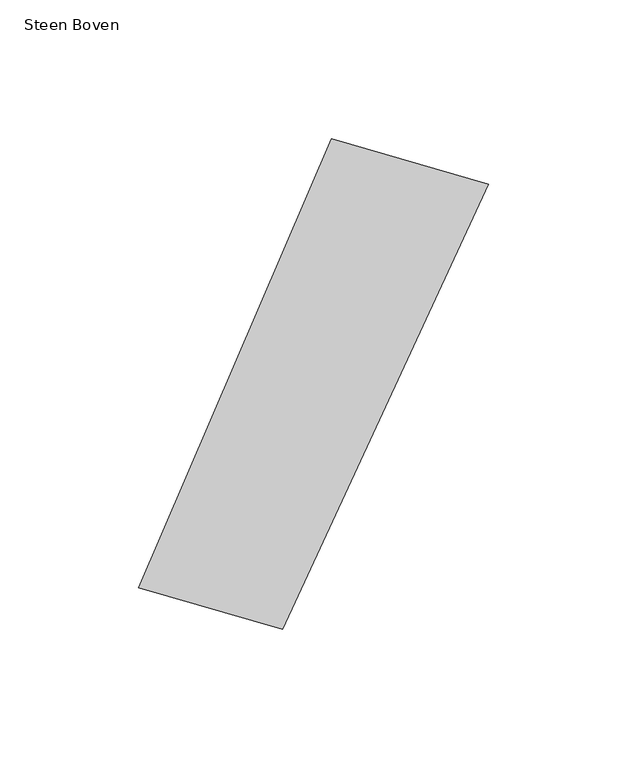
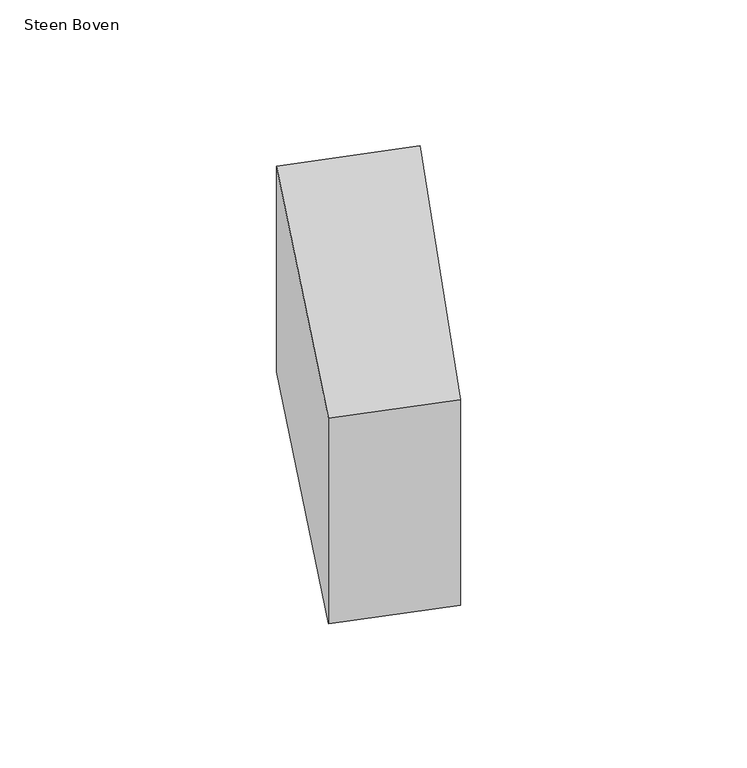
"""IFC4 building model written with IfcOpenShell, lengths in millimetres: proxy geometry, 00_GMA_steen_versie_4 : Steen Boven."""

import ifcopenshell
import ifcopenshell.guid

model = None  # the IFC model being written
_history = None  # IfcOwnerHistory: only IFC2X3 demands one
_inside = {}  # id of a spatial element -> (the spatial element, [elements in it])
_under = {}  # id of a project, library or spatial element -> (it, [spatial elements below it])
_declared = {}  # id of a project -> (the project, [libraries it declares])
_typed = {}  # id of a type object -> (the type object, [elements of that type])
_made_of = {}  # id of a material, layer set ... -> (it, [elements and type objects made of it])


def new_model(schema):
    """Start an empty IFC model of exactly this schema.

    Asked for "IFC4X3", IfcOpenShell would pick the latest addendum, in which some entities
    have other attributes; the version numbers below select the first issue.
    IFC2X3 requires an IfcOwnerHistory on every rooted entity: one is made here for all.
    """
    global model, _history
    if schema == "IFC4X3":
        model = ifcopenshell.file(schema_version=(4, 3, 0, 0))
    else:
        model = ifcopenshell.file(schema=schema)
    _inside.clear()
    _under.clear()
    _declared.clear()
    _typed.clear()
    _made_of.clear()
    _history = None
    if model.schema == "IFC2X3":
        org = make("IfcOrganization", Name="unknown")
        user = make(
            "IfcPersonAndOrganization",
            ThePerson=make("IfcPerson", FamilyName="unknown"),
            TheOrganization=org,
        )
        app = make(
            "IfcApplication",
            ApplicationDeveloper=org,
            Version="unknown",
            ApplicationFullName="unknown",
            ApplicationIdentifier="unknown",
        )
        _history = make(
            "IfcOwnerHistory",
            OwningUser=user,
            OwningApplication=app,
            ChangeAction="ADDED",
            CreationDate=0,
        )
    return model


def make(cls, **values):
    """One entity of the class cls with the attributes given. An attribute that is None is left unset."""
    return model.create_entity(
        cls, **{name: value for name, value in values.items() if value is not None}
    )


def rooted(cls, **values):
    """An entity with a GlobalId (a new one), such as an element, a storey or a relation."""
    return make(cls, GlobalId=ifcopenshell.guid.new(), OwnerHistory=_history, **values)


def si_unit(unit_type, name, prefix=None):
    """IfcSIUnit, for example si_unit("LENGTHUNIT", "METRE", prefix="MILLI")."""
    return make("IfcSIUnit", UnitType=unit_type, Prefix=prefix, Name=name)


def assignment(units):
    """IfcUnitAssignment: the units of a project."""
    return None if units is None else make("IfcUnitAssignment", Units=units)


def point(xyz):
    """IfcCartesianPoint."""
    return None if xyz is None else make("IfcCartesianPoint", Coordinates=xyz)


def direction(xyz):
    """IfcDirection."""
    return None if xyz is None else make("IfcDirection", DirectionRatios=xyz)


def frame(location, z_axis=None, x_axis=None):
    """IfcAxis2Placement3D, a coordinate frame: its origin and axes. An axis left out is left unset."""
    return make(
        "IfcAxis2Placement3D",
        Location=point(location),
        Axis=direction(z_axis),
        RefDirection=direction(x_axis),
    )


def origin():
    """The frame at (0, 0, 0) with its axes left unset."""
    return frame((0.0, 0.0, 0.0))


def origin_with_axes():
    """The frame at (0, 0, 0) with the z axis (0, 0, 1) and the x axis (1, 0, 0) written out."""
    return frame((0.0, 0.0, 0.0), z_axis=(0.0, 0.0, 1.0), x_axis=(1.0, 0.0, 0.0))


def place(relative_to, where):
    """IfcLocalPlacement: puts the frame where relative to a parent placement (None: the world)."""
    return make(
        "IfcLocalPlacement", PlacementRelTo=relative_to, RelativePlacement=where
    )


def context(
    kind, dimensions, precision=None, world=None, true_north=None, identifier=None
):
    """IfcGeometricRepresentationContext, for example the 3D "Model" context."""
    return make(
        "IfcGeometricRepresentationContext",
        ContextIdentifier=identifier,
        ContextType=kind,
        CoordinateSpaceDimension=dimensions,
        Precision=precision,
        WorldCoordinateSystem=world,
        TrueNorth=true_north,
    )


def project(units=None, contexts=None):
    """IfcProject with its units and contexts."""
    return rooted(
        "IfcProject",
        Name="project",
        RepresentationContexts=contexts,
        UnitsInContext=assignment(units),
    )


def spatial(cls, under=None, at=None, **own):
    """A site, building, storey or space (cls), placed at a placement, below another one or the project."""
    s = rooted(cls, ObjectPlacement=at, **own)
    if under is not None:
        _under.setdefault(under.id(), (under, []))[1].append(s)
    return s


def polyline(points):
    """IfcPolyline through the points."""
    return make("IfcPolyline", Points=[point(p) for p in points])


def outline(outer, holes=None, kind="AREA"):
    """IfcArbitraryClosedProfileDef: a profile drawn as a closed curve; with holes, ...WithVoids."""
    if holes is None:
        return make("IfcArbitraryClosedProfileDef", ProfileType=kind, OuterCurve=outer)
    return make(
        "IfcArbitraryProfileDefWithVoids",
        ProfileType=kind,
        OuterCurve=outer,
        InnerCurves=holes,
    )


def extrude(swept, where, along, depth):
    """IfcExtrudedAreaSolid: the profile swept, set in the frame where, extruded along a direction by depth."""
    return make(
        "IfcExtrudedAreaSolid",
        SweptArea=swept,
        Position=where,
        ExtrudedDirection=direction(along),
        Depth=depth,
    )


def shape(context_of_items, identifier, shape_type, items):
    """IfcShapeRepresentation: the items that make up one representation, for example the "Body"."""
    return make(
        "IfcShapeRepresentation",
        ContextOfItems=context_of_items,
        RepresentationIdentifier=identifier,
        RepresentationType=shape_type,
        Items=items,
    )


def source(mapping_origin, context_of_items, identifier, shape_type, items):
    """IfcRepresentationMap: a shape defined once, which mapped items show again and again."""
    return make(
        "IfcRepresentationMap",
        MappingOrigin=mapping_origin,
        MappedRepresentation=shape(context_of_items, identifier, shape_type, items),
    )


def transform(
    local_origin,
    x_axis=None,
    y_axis=None,
    z_axis=None,
    scale=None,
    scale2=None,
    scale3=None,
    uniform=True,
):
    """IfcCartesianTransformationOperator3D, or its non-uniform kind. x_axis, y_axis, z_axis: its Axis1, 2, 3."""
    if uniform:
        return make(
            "IfcCartesianTransformationOperator3D",
            Axis1=direction(x_axis),
            Axis2=direction(y_axis),
            LocalOrigin=point(local_origin),
            Scale=scale,
            Axis3=direction(z_axis),
        )
    return make(
        "IfcCartesianTransformationOperator3DnonUniform",
        Axis1=direction(x_axis),
        Axis2=direction(y_axis),
        LocalOrigin=point(local_origin),
        Scale=scale,
        Axis3=direction(z_axis),
        Scale2=scale2,
        Scale3=scale3,
    )


def mapped(mapping_source, mapping_target):
    """IfcMappedItem: shows the shape of a source again, moved by a transform."""
    return make(
        "IfcMappedItem", MappingSource=mapping_source, MappingTarget=mapping_target
    )


def made_of(thing, what):
    """Note that an element or type object is made of a material, layer set ...; save() writes the relation."""
    if what is not None:
        _made_of.setdefault(what.id(), (what, []))[1].append(thing)
    return thing


def element(
    cls,
    number,
    at=None,
    inside=None,
    cuts=None,
    type_object=None,
    material=None,
    context=None,
    identifier="Body",
    shape_type=None,
    held_by="IfcProductDefinitionShape",
    body=None,
    shapes=None,
    **own,
):
    """One element of the class cls, such as IfcWall. Its Tag is "e" and its number.

    at: its placement. inside: the storey or other place that contains it. cuts: it is an
    opening in that element (IfcRelVoidsElement). A single representation is given by context,
    identifier, shape_type and body (its items); several are given by shapes. held_by: the class
    of the entity that holds the representations. save() writes the other relations.
    """
    e = rooted(cls, Tag="e%d" % number, ObjectPlacement=at, **own)
    if body is not None:
        shapes = [shape(context, identifier, shape_type, body)]
    if shapes is not None:
        e.Representation = make(held_by, Representations=shapes)
    if inside is not None:
        _inside.setdefault(inside.id(), (inside, []))[1].append(e)
    if cuts is not None:
        rooted(
            "IfcRelVoidsElement", RelatingBuildingElement=cuts, RelatedOpeningElement=e
        )
    if type_object is not None:
        _typed.setdefault(type_object.id(), (type_object, []))[1].append(e)
    return made_of(e, material)


def aggregate(whole, parts):
    """IfcRelAggregates: a whole, such as a stair, and the parts it consists of."""
    return rooted("IfcRelAggregates", RelatingObject=whole, RelatedObjects=parts)


def save(model, path):
    """Write the relations noted so far, then the file.

    IfcRelAggregates (storeys below a building ...), IfcRelContainedInSpatialStructure (elements
    in a storey), IfcRelDefinesByType, IfcRelAssociatesMaterial and IfcRelDeclares: one each for
    every whole, place, type object, material and project.
    """
    for whole, parts in _under.values():
        aggregate(whole, parts)
    for where, things in _inside.values():
        rooted(
            "IfcRelContainedInSpatialStructure",
            RelatedElements=things,
            RelatingStructure=where,
        )
    for kind, things in _typed.values():
        rooted("IfcRelDefinesByType", RelatedObjects=things, RelatingType=kind)
    for what, things in _made_of.values():
        rooted("IfcRelAssociatesMaterial", RelatedObjects=things, RelatingMaterial=what)
    for by, libraries in _declared.values():
        rooted("IfcRelDeclares", RelatingContext=by, RelatedDefinitions=libraries)
    model.write(path)


def steen_boven_c7bab40e(model_context):
    return source(origin(), model_context, "Body", "SweptSolid", [
        extrude(outline(polyline([(138.9626949, 152.6124457), (64.6394864, -8.0916632), (12.6572251, 7.0193553), (82.3362997, 169.0557906), (138.9626949, 152.6124457)])), origin_with_axes(), (0.0, 0.0, 1.0), 100.0),
    ])


if __name__ == "__main__":
    model = new_model("IFC4")
    model_context = context("Model", 3, world=origin())
    ifc_project = project(units=[si_unit("LENGTHUNIT", "METRE", prefix="MILLI")], contexts=[model_context])
    site = spatial("IfcSite", under=ifc_project)
    building = spatial("IfcBuilding", under=site)
    placement = place(None, origin())
    steen_boven_shape = steen_boven_c7bab40e(model_context)
    element("IfcBuildingElementProxy", 1, Name="00_GMA_steen_versie_4 : Steen Boven", ObjectType="00_GMA_steen_versie_4 : Steen Boven", at=placement, inside=building, context=model_context, shape_type="MappedRepresentation", body=[
        mapped(steen_boven_shape, transform((0.0, 0.0, 0.0), x_axis=(1.0, 0.0, 0.0), y_axis=(0.0, 1.0, 0.0), z_axis=(0.0, 0.0, 1.0))),
    ])
    save(model, "model.ifc")

# Revit data of these elements
# Type "00_GMA_steen_versie_4 : Steen Boven"
#   StootVoegHalfBoven [instance default] = 5 mm
#   StootVoegHalf [instance default] = 5 mm
#   StootVoegBreedteOnder = 10 mm
#   StootVoegBreedteBoven = 10 mm
#   Steendikte = 100 mm
#   LintVoegOnderHalf = 5 mm
#   LintVoegOnder = 10 mm
#   LintVoegBovenHalf = 0 mm
#   LintVoegBoven = 0 mm
#   materiaal = none
#   MateriaalVoeg = none
#   Default Elevation = 0
